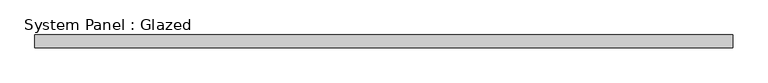
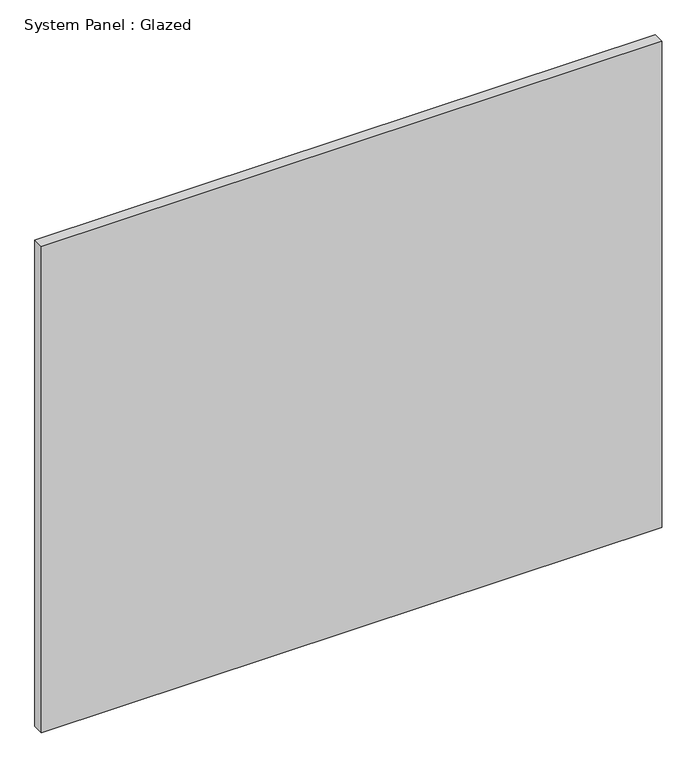
"""IFC4 building model written with IfcOpenShell, lengths in millimetres: plate geometry, System Panel : Glazed."""

from ifc_helpers import new_model, si_unit, origin, origin_with_axes, place, context, project, spatial, polyline, outline, extrude, source, transform, mapped, element, save


def system_panel_glazed_d25bfe26(model_context):
    return source(origin(), model_context, "Body", "SweptSolid", [
        extrude(outline(polyline([(697.4416668, -44.45), (-697.4416668, -44.45), (-697.4416668, -19.05), (697.4416668, -19.05), (697.4416668, -44.45)])), origin_with_axes(), (0.0, 0.0, 1.0), 1155.7),
    ])


if __name__ == "__main__":
    model = new_model("IFC4")
    model_context = context("Model", 3, world=origin())
    ifc_project = project(units=[si_unit("LENGTHUNIT", "METRE", prefix="MILLI")], contexts=[model_context])
    site = spatial("IfcSite", under=ifc_project)
    building = spatial("IfcBuilding", under=site)
    placement = place(None, origin())
    system_panel_glazed_shape = system_panel_glazed_d25bfe26(model_context)
    element("IfcPlate", 1, ObjectType="System Panel : Glazed", at=placement, inside=building, context=model_context, shape_type="MappedRepresentation", body=[
        mapped(system_panel_glazed_shape, transform((0.0, 0.0, 0.0), x_axis=(1.0, 0.0, 0.0), y_axis=(0.0, 1.0, 0.0), z_axis=(0.0, 0.0, 1.0))),
    ])
    save(model, "model.ifc")

# Revit data of these elements
# Type "System Panel : Glazed"
#   Construction Type Id = "GSP4R"
#   Analytic Construction = "1/8 in Pilkington single glazing"
#   Visual Light Transmittance = 0.9
#   Solar Heat Gain Coefficient = 0.86
#   Heat Transfer Coefficient (U) = 1.18115 BTU/(h·ft²·°F)
#   Define Thermal Properties by = 1
# Element 1 (IfcPlate, "System Panel : Glazed")
#   Materials on its faces: "Glass"
# Materials
#   "Glass": class "Glass", colour RGB 0 128 192, transparency 0.75, Description = "Soda Lime Glass", Cost = 0
